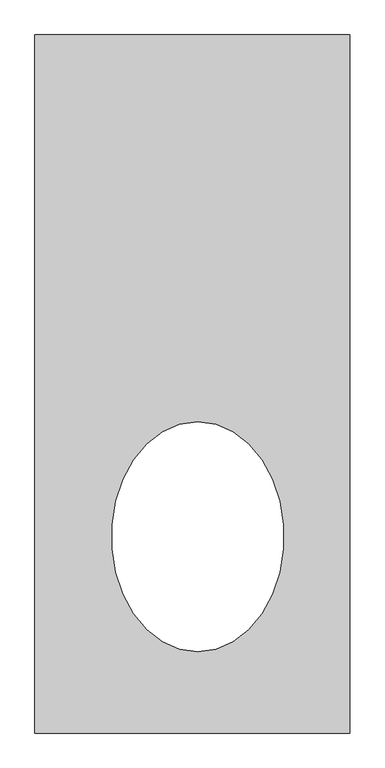
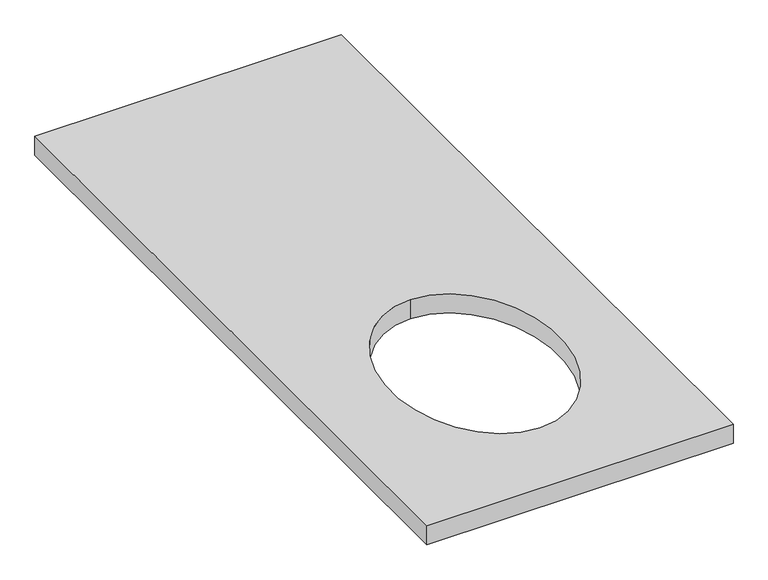
"""IFC4 building model written with IfcOpenShell, lengths in millimetres: furniture geometry, Master Bart - Counter 2 : Master Bart - Counter 2."""

from ifc_helpers import new_model, si_unit, point, frame, origin, place, context, project, spatial, ellipse_curve, trimmed, source, transform, mapped, element, save
from ifc_brep_helpers import plane_surface, extruded_surface, advanced_brep


def furniture_d44b89c1(model_context):
    return source(origin(), model_context, "Body", "AdvancedBrep", [
        advanced_brep(
        [(-6772.275, 13406.4375, 876.3), (-6772.275, 14693.9, 876.3), (-6191.25, 14693.9, 876.3), (-6191.25, 13406.4375, 876.3), (-6471.8449381, 13556.3938966, 876.3), (-6471.8449381, 13980.3938966, 876.3), (-6772.275, 13406.4375, 914.4), (-6191.25, 13406.4375, 914.4), (-6191.25, 14693.9, 914.4), (-6772.275, 14693.9, 914.4), (-6471.8449381, 13556.3938966, 914.4), (-6471.8449381, 13980.3938966, 914.4)],
        [
            (0, 1),
            (1, 2),
            (2, 3),
            (3, 0),
            (4, 5, ellipse_curve(frame((-6471.8449381, 13768.3938966, 876.3), z_axis=(0.0, 0.0, 1.0), x_axis=(0.0, 1.0, 0.0)), 212.0, 158.7697221)),
            (5, 4, ellipse_curve(frame((-6471.8449381, 13768.3938966, 876.3), z_axis=(0.0, 0.0, 1.0), x_axis=(0.0, 1.0, 0.0)), 212.0, 158.7697221)),
            (6, 7),
            (7, 8),
            (8, 9),
            (9, 6),
            (10, 11, ellipse_curve(frame((-6471.8449381, 13768.3938966, 914.4), z_axis=(0.0, 0.0, -1.0), x_axis=(0.0, 1.0, 0.0)), 212.0, 158.7697221)),
            (11, 10, ellipse_curve(frame((-6471.8449381, 13768.3938966, 914.4), z_axis=(0.0, 0.0, -1.0), x_axis=(0.0, 1.0, 0.0)), 212.0, 158.7697221)),
            (6, 0),
            (3, 7),
            (2, 8),
            (1, 9),
            (10, 4),
            (5, 11),
        ],
        [
            plane_surface(frame((-6207.4425, 13406.4375, 876.3), z_axis=(0.0, 0.0, -1.0), x_axis=(-1.0, 0.0, 0.0))),
            plane_surface(frame((-6207.4425, 13406.4375, 914.4), z_axis=(0.0, 0.0, 1.0), x_axis=(1.0, 0.0, 0.0))),
            plane_surface(frame((-6772.275, 13406.4375, 914.4), z_axis=(0.0, -1.0, 0.0), x_axis=(0.0, 0.0, -1.0))),
            plane_surface(frame((-6191.25, 13406.4375, 914.4), z_axis=(1.0, 0.0, 0.0), x_axis=(0.0, 0.0, -1.0))),
            plane_surface(frame((-6191.25, 14693.9, 914.4), z_axis=(0.0, 1.0, 0.0), x_axis=(0.0, 0.0, -1.0))),
            plane_surface(frame((-6772.275, 14693.9, 914.4), z_axis=(-1.0, 0.0, 0.0), x_axis=(0.0, 0.0, -1.0))),
            extruded_surface(trimmed(ellipse_curve(frame((-6471.8449381, 13768.3938966, -38.1), z_axis=(0.0, 0.0, -1.0), x_axis=(0.0, 1.0, 0.0)), 212.0, 158.7697221), [point((-6471.8449381, 13556.3938966, -38.1))], [point((-6471.8449381, 13980.3938966, -38.1))], True, "CARTESIAN"), (0.0, 0.0, 38.1), 38.1),
            extruded_surface(trimmed(ellipse_curve(frame((-6471.8449381, 13768.3938966, -38.1), z_axis=(0.0, 0.0, -1.0), x_axis=(0.0, 1.0, 0.0)), 212.0, 158.7697221), [point((-6471.8449381, 13980.3938966, -38.1))], [point((-6471.8449381, 13556.3938966, -38.1))], True, "CARTESIAN"), (0.0, 0.0, 38.1), 38.1),
        ],
        [
            (0, [[1, 2, 3, 4], [5, 6]]),
            (1, [[7, 8, 9, 10], [11, 12]]),
            (2, [[-7, 13, -4, 14]]),
            (3, [[-8, -14, -3, 15]]),
            (4, [[-9, -15, -2, 16]]),
            (5, [[-10, -16, -1, -13]]),
            (6, [[-11, 17, -6, 18]]),
            (7, [[-12, -18, -5, -17]]),
        ],
    ),
    ])


if __name__ == "__main__":
    model = new_model("IFC4")
    model_context = context("Model", 3, world=origin())
    ifc_project = project(units=[si_unit("LENGTHUNIT", "METRE", prefix="MILLI")], contexts=[model_context])
    site = spatial("IfcSite", under=ifc_project)
    building = spatial("IfcBuilding", under=site)
    placement = place(None, origin())
    furniture_shape = furniture_d44b89c1(model_context)
    element("IfcFurniture", 1, ObjectType="Master Bart - Counter 2 : Master Bart - Counter 2", at=placement, inside=building, context=model_context, shape_type="MappedRepresentation", body=[
        mapped(furniture_shape, transform((0.0, 0.0, 0.0), x_axis=(1.0, 0.0, 0.0), y_axis=(0.0, 1.0, 0.0), z_axis=(0.0, 0.0, 1.0))),
    ])
    save(model, "model.ifc")

# Revit data of these elements
# Type "Master Bart - Counter 2 : Master Bart - Counter 2"
#   COBie.Type = no
# Element 1 (IfcFurniture, "Master Bart - Counter 2 : Master Bart - Counter 2")
#   Materials on its faces: "Corian - Emerald"
# Materials
#   "Corian - Emerald": class "Plastic", colour RGB 51 95 44, transparency 0, Cost = 0
